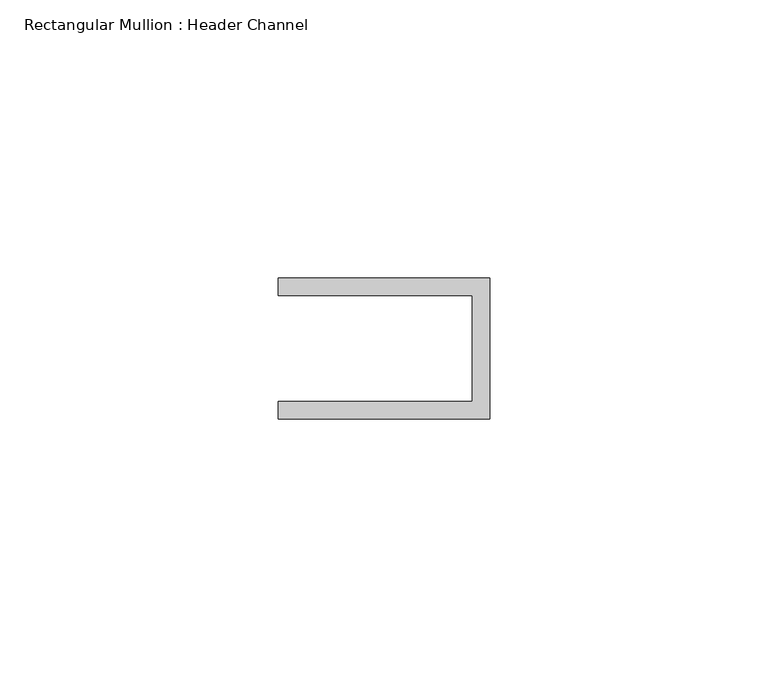
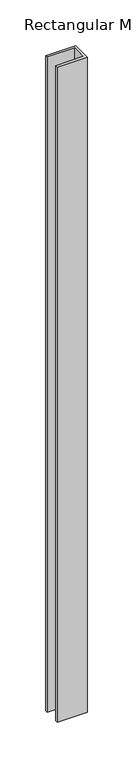
"""IFC4 building model written with IfcOpenShell, lengths in millimetres: member geometry, Rectangular Mullion : Header Channel."""

from ifc_helpers import new_model, si_unit, frame, origin, place, context, project, spatial, polyline, outline, extrude, source, transform, mapped, element, save


def rectangular_mullion_header_channel_d8f7347b(model_context):
    return source(origin(), model_context, "Body", "SweptSolid", [
        extrude(outline(polyline([(0.0, -12.7), (-38.1, -12.7), (-38.1, -9.525), (-3.175, -9.525), (-3.175, 9.525), (-38.1, 9.525), (-38.1, 12.7), (0.0, 12.7), (0.0, -12.7)])), frame((0.0, 0.0, -877.8332389), z_axis=(0.0, 0.0, 1.0), x_axis=(1.0, 0.0, 0.0)), (0.0, 0.0, 1.0), 877.8332389),
    ])


if __name__ == "__main__":
    model = new_model("IFC4")
    model_context = context("Model", 3, world=origin())
    ifc_project = project(units=[si_unit("LENGTHUNIT", "METRE", prefix="MILLI")], contexts=[model_context])
    site = spatial("IfcSite", under=ifc_project)
    building = spatial("IfcBuilding", under=site)
    placement = place(None, origin())
    rectangular_mullion_header_channel_shape = rectangular_mullion_header_channel_d8f7347b(model_context)
    element("IfcMember", 1, ObjectType="Rectangular Mullion : Header Channel", at=placement, inside=building, context=model_context, shape_type="MappedRepresentation", body=[
        mapped(rectangular_mullion_header_channel_shape, transform((0.0, 0.0, 0.0), x_axis=(1.0, 0.0, 0.0), y_axis=(0.0, 1.0, 0.0), z_axis=(0.0, 0.0, 1.0))),
    ])
    save(model, "model.ifc")

# Revit data of these elements
# Type "Rectangular Mullion : Header Channel"
#   built-in parameter 1007322 = 0.0833333 (stored number, unit not read)
#   built-in parameter 1007321 = -0.03125 (stored number, unit not read)
#   built-in parameter 1007320 = 0.0416667 (stored number, unit not read)
# Element 1 (IfcMember, "Rectangular Mullion : Header Channel")
#   Materials on its faces: "ALUM"
# Materials
#   "ALUM": class "Generic", colour RGB 157 157 157, transparency 0, Cost = 0
